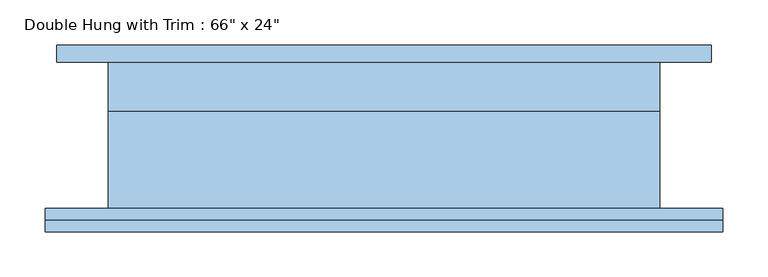
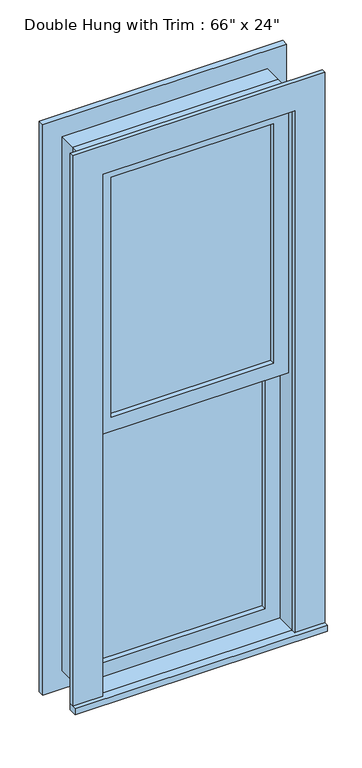
"""IFC4 building model written with IfcOpenShell, lengths in millimetres: window geometry."""

from ifc_helpers import new_model, si_unit, frame, origin, place, context, project, spatial, polyline, outline, extrude, source, transform, mapped, element, save


def window_9bb60c6b(model_context):
    return source(origin(), model_context, "Body", "SweptSolid", [
        extrude(outline(polyline([(-241.3, -1.5875), (-241.3, 11.1125), (241.3, 11.1125), (241.3, -1.5875), (-241.3, -1.5875)])), frame((0.0, 0.0, 977.9), z_axis=(0.0, 0.0, 1.0), x_axis=(1.0, 0.0, 0.0)), (0.0, 0.0, 1.0), 752.475),
        extrude(outline(polyline([(1774.825, -285.75), (933.45, -285.75), (933.45, 285.75), (1774.825, 285.75), (1774.825, -285.75)]), holes=[polyline([(1730.375, -241.3), (1730.375, 241.3), (977.9, 241.3), (977.9, -241.3), (1730.375, -241.3)])]), frame((0.0, -17.4625, 0.0), z_axis=(0.0, 1.0, 0.0), x_axis=(0.0, 0.0, 1.0)), (0.0, 0.0, 1.0), 44.45),
        extrude(outline(polyline([(-374.65, -106.3625), (-374.65, -80.9625), (374.65, -80.9625), (374.65, -106.3625), (-374.65, -106.3625)])), frame((0.0, 0.0, 914.4), z_axis=(0.0, 0.0, 1.0), x_axis=(1.0, 0.0, 0.0)), (0.0, 0.0, 1.0), 19.05),
        extrude(outline(polyline([(2571.75, -285.75), (2571.75, 285.75), (933.45, 285.75), (933.45, 374.65), (2660.65, 374.65), (2660.65, -374.65), (933.45, -374.65), (933.45, -285.75), (2571.75, -285.75)])), frame((0.0, -93.6625, 0.0), z_axis=(0.0, 1.0, 0.0), x_axis=(0.0, 0.0, 1.0)), (0.0, 0.0, 1.0), 12.7),
        extrude(outline(polyline([(2647.95, 361.95), (2647.95, -361.95), (857.25, -361.95), (857.25, 361.95), (2647.95, 361.95)]), holes=[polyline([(2559.05, 273.05), (946.15, 273.05), (946.15, -273.05), (2559.05, -273.05), (2559.05, 273.05)])]), frame((0.0, 80.9625, 0.0), z_axis=(0.0, 1.0, 0.0), x_axis=(0.0, 0.0, 1.0)), (0.0, 0.0, 1.0), 19.05),
        extrude(outline(polyline([(241.3, -33.3375), (241.3, -46.0375), (-241.3, -46.0375), (-241.3, -33.3375), (241.3, -33.3375)])), frame((0.0, 0.0, 1774.825), z_axis=(0.0, 0.0, 1.0), x_axis=(1.0, 0.0, 0.0)), (0.0, 0.0, 1.0), 752.475),
        extrude(outline(polyline([(2571.75, -285.75), (1730.375, -285.75), (1730.375, 285.75), (2571.75, 285.75), (2571.75, -285.75)]), holes=[polyline([(2527.3, -241.3), (2527.3, 241.3), (1774.825, 241.3), (1774.825, -241.3), (2527.3, -241.3)])]), frame((0.0, -61.9125, 0.0), z_axis=(0.0, 1.0, 0.0), x_axis=(0.0, 0.0, 1.0)), (0.0, 0.0, 1.0), 44.45),
        extrude(outline(polyline([(2590.8, -304.8), (914.4, -304.8), (914.4, 304.8), (2590.8, 304.8), (2590.8, -304.8)]), holes=[polyline([(2559.05, -273.05), (2559.05, 273.05), (946.15, 273.05), (946.15, -273.05), (2559.05, -273.05)])]), frame((0.0, 26.9875, 0.0), z_axis=(0.0, 1.0, 0.0), x_axis=(0.0, 0.0, 1.0)), (0.0, 0.0, 1.0), 53.975),
        extrude(outline(polyline([(2590.8, 304.8), (2590.8, -304.8), (914.4, -304.8), (914.4, 304.8), (2590.8, 304.8)]), holes=[polyline([(2571.75, 285.75), (933.45, 285.75), (933.45, -285.75), (2571.75, -285.75), (2571.75, 285.75)])]), frame((0.0, -80.9625, 0.0), z_axis=(0.0, 1.0, 0.0), x_axis=(0.0, 0.0, 1.0)), (0.0, 0.0, 1.0), 107.95),
    ])


if __name__ == "__main__":
    model = new_model("IFC4")
    model_context = context("Model", 3, world=origin())
    ifc_project = project(units=[si_unit("LENGTHUNIT", "METRE", prefix="MILLI")], contexts=[model_context])
    site = spatial("IfcSite", under=ifc_project)
    building = spatial("IfcBuilding", under=site)
    placement = place(None, origin())
    window_shape = window_9bb60c6b(model_context)
    element("IfcWindow", 1, ObjectType="Double Hung with Trim : 66\" x 24\"", at=placement, inside=building, context=model_context, shape_type="MappedRepresentation", body=[
        mapped(window_shape, transform((0.0, 0.0, 0.0), x_axis=(1.0, 0.0, 0.0), y_axis=(0.0, 1.0, 0.0), z_axis=(0.0, 0.0, 1.0))),
    ])
    save(model, "model.ifc")

# Revit data of these elements
# Type "Double Hung with Trim : 66\" x 24\""
#   Type Mark = "44"
#   COBie.Type.CreatedBy = "doug.wood@us.ibm.com"
#   COBie.Type.CreatedOn = "2016-04-14T02:07:26"
#   COBie.Type.Name = "Windows_Double Hung with Trim_66\" x 24\"_44"
#   COBie.Type.Category = "23-30 20 17 17 14 : Double-Hung Windows"
#   COBie.Type.Description = "Double Hung with Trim_66\" x 24\""
#   COBie.Type.Manufacturer = ""
#   COBie.Type.ModelNumber = ""
#   Construction Type Id = "GSP4R"
#   Assembly Code = "B2020100"
#   Analytic Construction = "1/8 in Pilkington single glazing"
#   COBie.Type.ReplacementCost = 0
#   Visual Light Transmittance = 0.9
#   Solar Heat Gain Coefficient = 0.78
#   Heat Transfer Coefficient (U) = 3.6886 W/(m²·K)
#   Height = 5' - 6"
#   Default Sill Height = 3' - 0"
#   Trim Projection - Ext. = 0' - 0 1/2"
#   Trim Projection - Int. = 0' - 0 3/4"
#   Trim Width - Exterior = 0' - 3 1/2"
#   Trim Width - Interior = 0' - 3 1/2"
#   Width = 2' - 0"
#   Window Inset = 0' - 0 3/4"
#   COBie.Type = no
#   Glass Pane Material = Glass
#   Sash Material = Sash - White
#   Trim Exterior Material = Trim - White
#   Trim Interior Material = Trim - White
#   Wall Closure = (empty or 0)
# Element 1 (IfcWindow, "Double Hung with Trim : 66\" x 24\"")
#   Materials on its faces: "Sash - White", "Trim - White", "Glass"
# Materials
#   "Glass": class "Glass", colour RGB 0 128 192, transparency 0.75, Description = "Soda Lime Glass", Cost = 0
#   "Sash - White": class "Wood", colour RGB 255 255 255, transparency 0, Cost = 0
#   "Trim - White": class "Wood", colour RGB 255 255 255, transparency 0, Cost = 0
